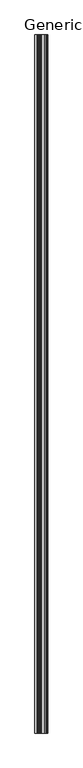
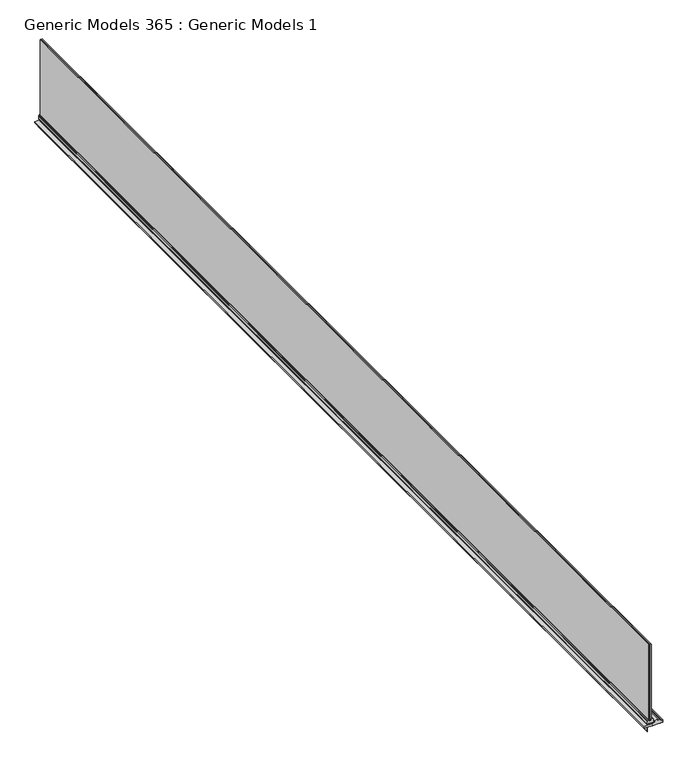
"""IFC4 building model written with IfcOpenShell, lengths in millimetres: proxy geometry, Generic Models 365 : Generic Models 1."""

import ifcopenshell
import ifcopenshell.guid

model = None  # the IFC model being written
_history = None  # IfcOwnerHistory: only IFC2X3 demands one
_inside = {}  # id of a spatial element -> (the spatial element, [elements in it])
_under = {}  # id of a project, library or spatial element -> (it, [spatial elements below it])
_declared = {}  # id of a project -> (the project, [libraries it declares])
_typed = {}  # id of a type object -> (the type object, [elements of that type])
_made_of = {}  # id of a material, layer set ... -> (it, [elements and type objects made of it])


def new_model(schema):
    """Start an empty IFC model of exactly this schema.

    Asked for "IFC4X3", IfcOpenShell would pick the latest addendum, in which some entities
    have other attributes; the version numbers below select the first issue.
    IFC2X3 requires an IfcOwnerHistory on every rooted entity: one is made here for all.
    """
    global model, _history
    if schema == "IFC4X3":
        model = ifcopenshell.file(schema_version=(4, 3, 0, 0))
    else:
        model = ifcopenshell.file(schema=schema)
    _inside.clear()
    _under.clear()
    _declared.clear()
    _typed.clear()
    _made_of.clear()
    _history = None
    if model.schema == "IFC2X3":
        org = make("IfcOrganization", Name="unknown")
        user = make(
            "IfcPersonAndOrganization",
            ThePerson=make("IfcPerson", FamilyName="unknown"),
            TheOrganization=org,
        )
        app = make(
            "IfcApplication",
            ApplicationDeveloper=org,
            Version="unknown",
            ApplicationFullName="unknown",
            ApplicationIdentifier="unknown",
        )
        _history = make(
            "IfcOwnerHistory",
            OwningUser=user,
            OwningApplication=app,
            ChangeAction="ADDED",
            CreationDate=0,
        )
    return model


def make(cls, **values):
    """One entity of the class cls with the attributes given. An attribute that is None is left unset."""
    return model.create_entity(
        cls, **{name: value for name, value in values.items() if value is not None}
    )


def rooted(cls, **values):
    """An entity with a GlobalId (a new one), such as an element, a storey or a relation."""
    return make(cls, GlobalId=ifcopenshell.guid.new(), OwnerHistory=_history, **values)


def si_unit(unit_type, name, prefix=None):
    """IfcSIUnit, for example si_unit("LENGTHUNIT", "METRE", prefix="MILLI")."""
    return make("IfcSIUnit", UnitType=unit_type, Prefix=prefix, Name=name)


def assignment(units):
    """IfcUnitAssignment: the units of a project."""
    return None if units is None else make("IfcUnitAssignment", Units=units)


def point(xyz):
    """IfcCartesianPoint."""
    return None if xyz is None else make("IfcCartesianPoint", Coordinates=xyz)


def direction(xyz):
    """IfcDirection."""
    return None if xyz is None else make("IfcDirection", DirectionRatios=xyz)


def frame(location, z_axis=None, x_axis=None):
    """IfcAxis2Placement3D, a coordinate frame: its origin and axes. An axis left out is left unset."""
    return make(
        "IfcAxis2Placement3D",
        Location=point(location),
        Axis=direction(z_axis),
        RefDirection=direction(x_axis),
    )


def frame_2d(location, x_axis=None):
    """IfcAxis2Placement2D, a coordinate frame in the plane: its origin and x axis."""
    return make(
        "IfcAxis2Placement2D", Location=point(location), RefDirection=direction(x_axis)
    )


def origin():
    """The frame at (0, 0, 0) with its axes left unset."""
    return frame((0.0, 0.0, 0.0))


def place(relative_to, where):
    """IfcLocalPlacement: puts the frame where relative to a parent placement (None: the world)."""
    return make(
        "IfcLocalPlacement", PlacementRelTo=relative_to, RelativePlacement=where
    )


def context(
    kind, dimensions, precision=None, world=None, true_north=None, identifier=None
):
    """IfcGeometricRepresentationContext, for example the 3D "Model" context."""
    return make(
        "IfcGeometricRepresentationContext",
        ContextIdentifier=identifier,
        ContextType=kind,
        CoordinateSpaceDimension=dimensions,
        Precision=precision,
        WorldCoordinateSystem=world,
        TrueNorth=true_north,
    )


def project(units=None, contexts=None):
    """IfcProject with its units and contexts."""
    return rooted(
        "IfcProject",
        Name="project",
        RepresentationContexts=contexts,
        UnitsInContext=assignment(units),
    )


def spatial(cls, under=None, at=None, **own):
    """A site, building, storey or space (cls), placed at a placement, below another one or the project."""
    s = rooted(cls, ObjectPlacement=at, **own)
    if under is not None:
        _under.setdefault(under.id(), (under, []))[1].append(s)
    return s


def polyline(points):
    """IfcPolyline through the points."""
    return make("IfcPolyline", Points=[point(p) for p in points])


def circle_curve(where, radius):
    """IfcCircle in the frame where."""
    return make("IfcCircle", Position=where, Radius=radius)


def trimmed(basis, trim1, trim2, sense, master):
    """IfcTrimmedCurve: the piece of a basis curve between two trims."""
    return make(
        "IfcTrimmedCurve",
        BasisCurve=basis,
        Trim1=trim1,
        Trim2=trim2,
        SenseAgreement=sense,
        MasterRepresentation=master,
    )


def segment(curve, same_sense, transition):
    """IfcCompositeCurveSegment."""
    return make(
        "IfcCompositeCurveSegment",
        Transition=transition,
        SameSense=same_sense,
        ParentCurve=curve,
    )


def composite_curve(segments, self_intersect=None):
    """IfcCompositeCurve: segments joined end to end."""
    return make("IfcCompositeCurve", Segments=segments, SelfIntersect=self_intersect)


def outline(outer, holes=None, kind="AREA"):
    """IfcArbitraryClosedProfileDef: a profile drawn as a closed curve; with holes, ...WithVoids."""
    if holes is None:
        return make("IfcArbitraryClosedProfileDef", ProfileType=kind, OuterCurve=outer)
    return make(
        "IfcArbitraryProfileDefWithVoids",
        ProfileType=kind,
        OuterCurve=outer,
        InnerCurves=holes,
    )


def extrude(swept, where, along, depth):
    """IfcExtrudedAreaSolid: the profile swept, set in the frame where, extruded along a direction by depth."""
    return make(
        "IfcExtrudedAreaSolid",
        SweptArea=swept,
        Position=where,
        ExtrudedDirection=direction(along),
        Depth=depth,
    )


def shape(context_of_items, identifier, shape_type, items):
    """IfcShapeRepresentation: the items that make up one representation, for example the "Body"."""
    return make(
        "IfcShapeRepresentation",
        ContextOfItems=context_of_items,
        RepresentationIdentifier=identifier,
        RepresentationType=shape_type,
        Items=items,
    )


def source(mapping_origin, context_of_items, identifier, shape_type, items):
    """IfcRepresentationMap: a shape defined once, which mapped items show again and again."""
    return make(
        "IfcRepresentationMap",
        MappingOrigin=mapping_origin,
        MappedRepresentation=shape(context_of_items, identifier, shape_type, items),
    )


def transform(
    local_origin,
    x_axis=None,
    y_axis=None,
    z_axis=None,
    scale=None,
    scale2=None,
    scale3=None,
    uniform=True,
):
    """IfcCartesianTransformationOperator3D, or its non-uniform kind. x_axis, y_axis, z_axis: its Axis1, 2, 3."""
    if uniform:
        return make(
            "IfcCartesianTransformationOperator3D",
            Axis1=direction(x_axis),
            Axis2=direction(y_axis),
            LocalOrigin=point(local_origin),
            Scale=scale,
            Axis3=direction(z_axis),
        )
    return make(
        "IfcCartesianTransformationOperator3DnonUniform",
        Axis1=direction(x_axis),
        Axis2=direction(y_axis),
        LocalOrigin=point(local_origin),
        Scale=scale,
        Axis3=direction(z_axis),
        Scale2=scale2,
        Scale3=scale3,
    )


def mapped(mapping_source, mapping_target):
    """IfcMappedItem: shows the shape of a source again, moved by a transform."""
    return make(
        "IfcMappedItem", MappingSource=mapping_source, MappingTarget=mapping_target
    )


def made_of(thing, what):
    """Note that an element or type object is made of a material, layer set ...; save() writes the relation."""
    if what is not None:
        _made_of.setdefault(what.id(), (what, []))[1].append(thing)
    return thing


def element(
    cls,
    number,
    at=None,
    inside=None,
    cuts=None,
    type_object=None,
    material=None,
    context=None,
    identifier="Body",
    shape_type=None,
    held_by="IfcProductDefinitionShape",
    body=None,
    shapes=None,
    **own,
):
    """One element of the class cls, such as IfcWall. Its Tag is "e" and its number.

    at: its placement. inside: the storey or other place that contains it. cuts: it is an
    opening in that element (IfcRelVoidsElement). A single representation is given by context,
    identifier, shape_type and body (its items); several are given by shapes. held_by: the class
    of the entity that holds the representations. save() writes the other relations.
    """
    e = rooted(cls, Tag="e%d" % number, ObjectPlacement=at, **own)
    if body is not None:
        shapes = [shape(context, identifier, shape_type, body)]
    if shapes is not None:
        e.Representation = make(held_by, Representations=shapes)
    if inside is not None:
        _inside.setdefault(inside.id(), (inside, []))[1].append(e)
    if cuts is not None:
        rooted(
            "IfcRelVoidsElement", RelatingBuildingElement=cuts, RelatedOpeningElement=e
        )
    if type_object is not None:
        _typed.setdefault(type_object.id(), (type_object, []))[1].append(e)
    return made_of(e, material)


def aggregate(whole, parts):
    """IfcRelAggregates: a whole, such as a stair, and the parts it consists of."""
    return rooted("IfcRelAggregates", RelatingObject=whole, RelatedObjects=parts)


def save(model, path):
    """Write the relations noted so far, then the file.

    IfcRelAggregates (storeys below a building ...), IfcRelContainedInSpatialStructure (elements
    in a storey), IfcRelDefinesByType, IfcRelAssociatesMaterial and IfcRelDeclares: one each for
    every whole, place, type object, material and project.
    """
    for whole, parts in _under.values():
        aggregate(whole, parts)
    for where, things in _inside.values():
        rooted(
            "IfcRelContainedInSpatialStructure",
            RelatedElements=things,
            RelatingStructure=where,
        )
    for kind, things in _typed.values():
        rooted("IfcRelDefinesByType", RelatedObjects=things, RelatingType=kind)
    for what, things in _made_of.values():
        rooted("IfcRelAssociatesMaterial", RelatedObjects=things, RelatingMaterial=what)
    for by, libraries in _declared.values():
        rooted("IfcRelDeclares", RelatingContext=by, RelatedDefinitions=libraries)
    model.write(path)


def generic_models_365_generic_models_1_1044130a(model_context):
    return source(origin(), model_context, "Body", "SweptSolid", [
        extrude(outline(composite_curve([segment(polyline([(125550.1321292, -15554.6966554), (125558.0823465, -15554.6966554), (125558.0823465, -15562.6468485), (125560.063524, -15562.6468485), (125560.063524, -15554.6966554), (125569.994943, -15554.6966554), (125569.994943, -15565.0090105), (125570.8077325, -15565.7964624), (125570.8077325, -15568.9714624), (125574.770136, -15568.9714624), (125574.770136, -15570.5716554), (125577.945136, -15574.5086244), (125577.945136, -15576.1088175), (125580.3327325, -15576.1088175), (125580.3327325, -15595.1588175), (125586.664565, -15595.1588175), (125586.664565, -15624.5720415), (125583.489565, -15624.5720415), (125583.489565, -15621.5240686), (125574.802765, -15621.5240686), (125574.802765, -15603.9980686), (125572.516765, -15603.9980686), (125572.516765, -15621.5240686), (125571.5769685, -15621.5240686), (125571.5769685, -15629.9314043), (125563.6267755, -15629.9314043), (125563.6267755, -15631.9126787), (125570.0457151, -15631.9126787), (125570.0457151, -15635.9258058), (125565.1689224, -15635.9258058), (125565.1689224, -15670.8762058), (125562.7465526, -15698.7400058), (125553.8151292, -15698.7400058), (125553.8151292, -15690.8364402), (125551.5291292, -15690.8364402), (125551.5291292, -15697.1864402), (125550.1321292, -15697.1864402), (125550.1321292, -15672.2986058), (125514.7650422, -15672.2986058)]), True, "CONTINUOUS"), segment(trimmed(circle_curve(frame_2d((125514.7625825, -15671.600106)), 0.6985041), [point((125514.7650422, -15672.2986058))], [point((125514.7602416, -15670.9016058))], False, "CARTESIAN"), True, "CONTINUOUS"), segment(polyline([(125514.7602416, -15670.9016058), (125550.1321292, -15670.9016058), (125550.1321292, -15634.432438), (125553.3071292, -15634.432438), (125553.3071292, -15632.146438), (125550.1321292, -15632.146438), (125550.1321292, -15615.0470554), (125552.2149292, -15615.0470554), (125552.2149292, -15611.8720554), (125550.1321292, -15611.8720554), (125550.1321292, -15594.8449558), (125553.3071292, -15594.8449558), (125553.3071292, -15592.5589519), (125550.1321292, -15592.5589519), (125550.1321292, -15575.0512027), (125553.3071292, -15575.0512027), (125553.3071292, -15572.7651989), (125550.1321292, -15572.7651989), (125550.1321292, -15554.6966554)]), True, "CONTINUOUS")], self_intersect=False)), frame((0.0, 306.6963299, 0.0), z_axis=(0.0, 1.0, 0.0), x_axis=(0.0, 0.0, 1.0)), (0.0, 0.0, 1.0), 7886.7),
        extrude(outline(composite_curve([segment(polyline([(125598.9890401, -15662.3997479), (125603.2244792, -15662.3997479), (125603.2244792, -15663.5356058), (125605.2508531, -15663.5356058), (125605.0613027, -15665.9786453), (125597.2554792, -15668.5140058), (125597.2554792, -15670.9016058), (125574.9542792, -15670.9016058)]), True, "CONTINUOUS"), segment(trimmed(circle_curve(frame_2d((125574.9542792, -15668.5140058)), 2.3876), [point((125574.9542792, -15670.9016058))], [point((125572.5666792, -15668.5140058))], False, "CARTESIAN"), True, "CONTINUOUS"), segment(polyline([(125572.5666792, -15668.5140058), (125572.5666792, -15665.9486058), (125574.5986792, -15665.9486058), (125574.5986792, -15664.2722058), (125577.9006792, -15664.2722058), (125577.9006792, -15662.3672058), (125569.9758792, -15662.3672058), (125569.9758792, -15656.7538058), (125575.2844792, -15656.7538058), (125575.2844792, -15644.5618058)]), True, "CONTINUOUS"), segment(trimmed(circle_curve(frame_2d((125575.2844792, -15642.5806058)), 1.9812), [point((125575.2844792, -15644.5618058))], [point((125575.2844792, -15640.5994058))], True, "CARTESIAN"), True, "CONTINUOUS"), segment(polyline([(125575.2844792, -15640.5994058), (125575.2844792, -15627.2644058)]), True, "CONTINUOUS"), segment(trimmed(circle_curve(frame_2d((125576.0972792, -15627.2644058)), 0.8128), [point((125575.2844792, -15627.2644058))], [point((125576.0972792, -15626.4516058))], False, "CARTESIAN"), True, "CONTINUOUS"), segment(polyline([(125576.0972792, -15626.4516058), (125594.3852792, -15626.4516058), (125594.3852792, -15628.3321238), (125595.986168, -15628.3321238), (125595.986168, -15626.7319238), (125603.529968, -15626.7319238), (125603.529968, -15630.4998433), (125605.692318, -15630.4998433), (125606.704968, -15642.3275238), (125596.773568, -15642.3275238), (125594.3852792, -15639.939235), (125594.3852792, -15661.3766058), (125597.965898, -15661.3766058), (125598.9890401, -15662.3997479)]), True, "CONTINUOUS")], self_intersect=False)), frame((0.0, 306.6963299, 0.0), z_axis=(0.0, 1.0, 0.0), x_axis=(0.0, 0.0, 1.0)), (0.0, 0.0, 1.0), 7886.7),
        extrude(outline(polyline([(-15643.1212738, 306.6963299), (-15647.8837738, 306.6963299), (-15647.8837738, 8193.3963299), (-15643.1212738, 8193.3963299), (-15643.1212738, 306.6963299)])), frame((0.0, 0.0, 125595.1790292), z_axis=(0.0, 0.0, 1.0), x_axis=(1.0, 0.0, 0.0)), (0.0, 0.0, 1.0), 602.3375481),
        extrude(outline(polyline([(-15648.6775238, 306.6963299), (-15655.0266058, 306.6963299), (-15655.0266058, 8193.3963299), (-15648.6775238, 8193.3963299), (-15648.6775238, 306.6963299)])), frame((0.0, 0.0, 125595.1790292), z_axis=(0.0, 0.0, 1.0), x_axis=(1.0, 0.0, 0.0)), (0.0, 0.0, 1.0), 6.35),
        extrude(outline(polyline([(-15655.8203558, 306.6963299), (-15660.5828558, 306.6963299), (-15660.5828558, 8193.3963299), (-15655.8203558, 8193.3963299), (-15655.8203558, 306.6963299)])), frame((0.0, 0.0, 125595.1790292), z_axis=(0.0, 0.0, 1.0), x_axis=(1.0, 0.0, 0.0)), (0.0, 0.0, 1.0), 602.3375481),
    ])


if __name__ == "__main__":
    model = new_model("IFC4")
    model_context = context("Model", 3, world=origin())
    ifc_project = project(units=[si_unit("LENGTHUNIT", "METRE", prefix="MILLI")], contexts=[model_context])
    site = spatial("IfcSite", under=ifc_project)
    building = spatial("IfcBuilding", under=site)
    placement = place(None, origin())
    generic_models_365_generic_models_1_shape = generic_models_365_generic_models_1_1044130a(model_context)
    element("IfcBuildingElementProxy", 1, Name="Generic Models 365 : Generic Models 1", ObjectType="Generic Models 365 : Generic Models 1", at=placement, inside=building, context=model_context, shape_type="MappedRepresentation", body=[
        mapped(generic_models_365_generic_models_1_shape, transform((0.0, 0.0, 0.0), x_axis=(1.0, 0.0, 0.0), y_axis=(0.0, 1.0, 0.0), z_axis=(0.0, 0.0, 1.0))),
    ])
    save(model, "model.ifc")

# Revit data of these elements
# Element 1 (IfcBuildingElementProxy, "Generic Models 365 : Generic Models 1")
#   Materials on its faces: "_WINDOW PER SCHEDULE"
# Materials
#   "_WINDOW PER SCHEDULE": class "Generic", colour RGB 255 255 255, transparency 0, Cost = 0
